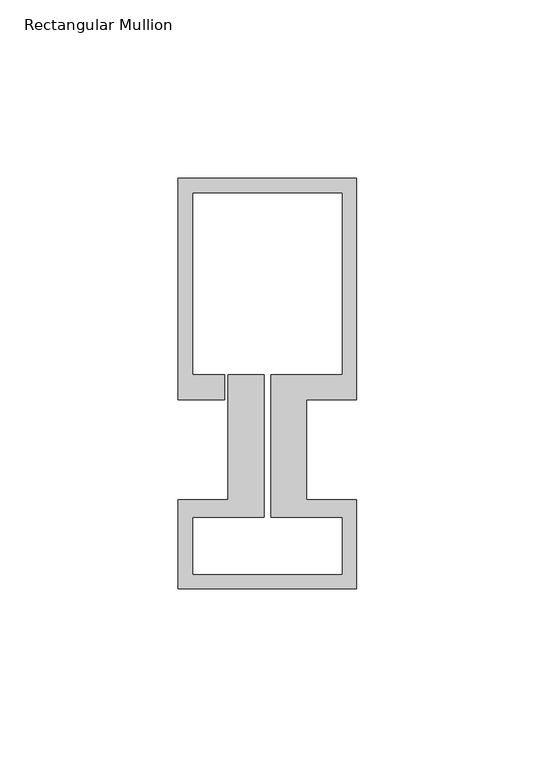
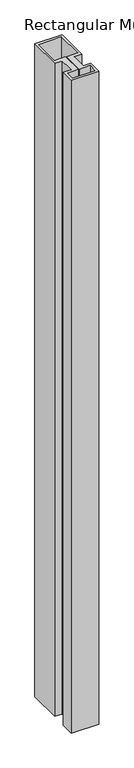
"""IFC4 building model written with IfcOpenShell, lengths in millimetres: member geometry, Rectangular Mullion : Schueco_FWS-50-HI_Tran_CovCap-20mm_Tran-55mm."""

from ifc_helpers import new_model, si_unit, frame, origin, place, context, project, spatial, polyline, outline, extrude, source, transform, mapped, element, save


def rectangular_mullion_19d93d62(model_context):
    return source(origin(), model_context, "Body", "SweptSolid", [
        extrude(outline(polyline([(0.0, 90.0), (0.0, 28.0), (-14.0, 28.0), (-14.0, -0.1), (0.0, -0.1), (0.0, -25.0), (-50.0, -25.0), (-50.0, -0.1), (-36.0, -0.1), (-36.0, 35.0), (-26.0, 35.0), (-26.0, -5.0), (-46.0, -5.0), (-46.0, -21.0), (-4.0, -21.0), (-4.0, -5.0), (-24.0, -5.0), (-24.0, 35.0), (-4.0, 35.0), (-4.0, 86.0), (-46.0, 86.0), (-46.0, 35.0), (-37.0, 35.0), (-37.0, 28.0), (-50.0, 28.0), (-50.0, 90.0), (0.0, 90.0)])), frame((0.0, 0.0, -1260.0), z_axis=(0.0, 0.0, 1.0), x_axis=(1.0, 0.0, 0.0)), (0.0, 0.0, 1.0), 1260.0),
    ])


if __name__ == "__main__":
    model = new_model("IFC4")
    model_context = context("Model", 3, world=origin())
    ifc_project = project(units=[si_unit("LENGTHUNIT", "METRE", prefix="MILLI")], contexts=[model_context])
    site = spatial("IfcSite", under=ifc_project)
    building = spatial("IfcBuilding", under=site)
    placement = place(None, origin())
    rectangular_mullion_shape = rectangular_mullion_19d93d62(model_context)
    element("IfcMember", 1, ObjectType="Rectangular Mullion : Schueco_FWS-50-HI_Tran_CovCap-20mm_Tran-55mm", at=placement, inside=building, context=model_context, shape_type="MappedRepresentation", body=[
        mapped(rectangular_mullion_shape, transform((0.0, 0.0, 0.0), x_axis=(1.0, 0.0, 0.0), y_axis=(0.0, 1.0, 0.0), z_axis=(0.0, 0.0, 1.0))),
    ])
    save(model, "model.ifc")

# Revit data of these elements
# Type "Rectangular Mullion : Schueco_FWS-50-HI_Tran_CovCap-20mm_Tran-55mm"
#   Model = "FWS 50.HI"
#   Manufacturer = "Schueco International KG"
#   Type Comments = "Transom"
#   Schueco thermal insulation standard = "Highly thermally insulated"
#   Burglar resistance = "RC 3"
#   Thermal insulation = "to 0.90 W/(m²K)"
#   built-in parameter 1007322 = 0.377297 (stored number, unit not read)
#   built-in parameter 1007321 = 0.0360892 (stored number, unit not read)
#   built-in parameter 1007320 = 0.0360892 (stored number, unit not read)
# Element 1 (IfcMember, "Rectangular Mullion : Schueco_FWS-50-HI_Tran_CovCap-20mm_Tran-55mm")
#   Materials on its faces: "Alu"
# Materials
#   "Alu": class "Glas", colour RGB 140 140 140, transparency 0
